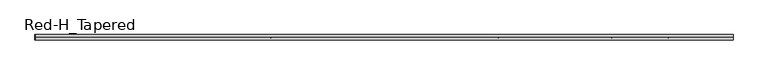
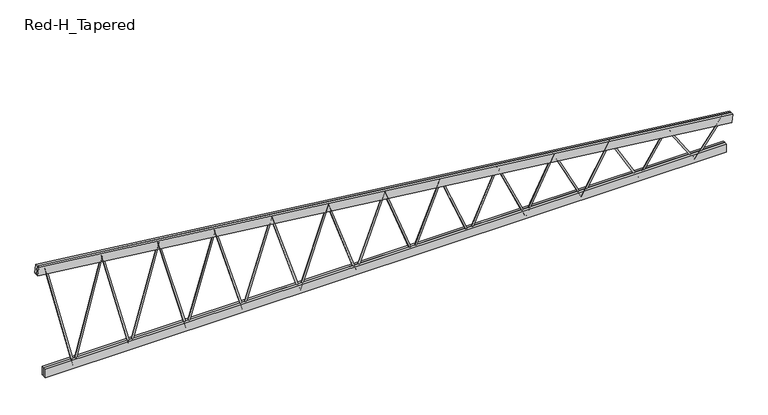
"""IFC4 building model written with IfcOpenShell, lengths in millimetres: beam geometry, Construction_Frames_RedBuilt_Openweb_Red-H_Tapered : Red-H_Tapered."""

from ifc_helpers import new_model, si_unit, point, frame, origin, origin_2d, place, context, project, spatial, polyline, circle_curve, trimmed, segment, composite_curve, outline, extrude, source, transform, mapped, element, save


def red_h_tapered_f2622887(model_context):
    return source(origin(), model_context, "Body", "SweptSolid", [
        extrude(outline(composite_curve([segment(trimmed(circle_curve(origin_2d(), 12.7), [point((0.0, -12.7000001))], [point((0.0, 12.6999999))], False, "CARTESIAN"), True, "CONTINUOUS"), segment(trimmed(circle_curve(origin_2d(), 12.7), [point((0.0, 12.6999999))], [point((0.0, -12.7000001))], False, "CARTESIAN"), True, "CONTINUOUS")], self_intersect=False)), frame((-450.1223958, 0.0, -367.0101562), z_axis=(-0.32912844274512754, 0.0, 0.9442851625309843), x_axis=(0.0, -1.0, 0.0)), (0.0, 0.0, 1.0), 1367.6192555),
        extrude(outline(composite_curve([segment(trimmed(circle_curve(origin_2d(), 12.7), [point((0.0, 12.7000001))], [point((0.0, -12.7))], False, "CARTESIAN"), True, "CONTINUOUS"), segment(trimmed(circle_curve(origin_2d(), 12.7), [point((0.0, -12.7))], [point((0.0, 12.7000001))], False, "CARTESIAN"), True, "CONTINUOUS")], self_intersect=False)), frame((-1350.3671875, 0.0, -367.0101562), z_axis=(0.3291284427451277, 0.0, 0.9442851625309842), x_axis=(0.0, -1.0, 0.0)), (0.0, 0.0, 1.0), 1367.6192555),
        extrude(outline(composite_curve([segment(trimmed(circle_curve(origin_2d(), 12.7), [point((0.0, -12.7))], [point((0.0, 12.7))], False, "CARTESIAN"), True, "CONTINUOUS"), segment(trimmed(circle_curve(origin_2d(), 12.7), [point((0.0, 12.7))], [point((0.0, -12.7))], False, "CARTESIAN"), True, "CONTINUOUS")], self_intersect=False)), frame((-1350.3671875, 0.0, -367.0101562), z_axis=(-0.3075867291849269, 0.0, 0.9515200491998677), x_axis=(0.0, -1.0, 0.0)), (0.0, 0.0, 1.0), 1463.3999231),
        extrude(outline(composite_curve([segment(trimmed(circle_curve(origin_2d(), 12.7), [point((0.0, -12.7))], [point((0.0, 12.7000001))], False, "CARTESIAN"), True, "CONTINUOUS"), segment(trimmed(circle_curve(origin_2d(), 12.7), [point((0.0, 12.7000001))], [point((0.0, -12.7))], False, "CARTESIAN"), True, "CONTINUOUS")], self_intersect=False)), frame((-2250.6119792, 0.0, -367.0101562), z_axis=(0.3075867291849308, 0.0, 0.9515200491998664), x_axis=(0.0, -1.0, 0.0)), (0.0, 0.0, 1.0), 1463.3999231),
        extrude(outline(composite_curve([segment(trimmed(circle_curve(origin_2d(), 12.7), [point((0.0, 12.7))], [point((0.0, -12.7))], False, "CARTESIAN"), True, "CONTINUOUS"), segment(trimmed(circle_curve(origin_2d(), 12.7), [point((0.0, -12.7))], [point((0.0, 12.7))], False, "CARTESIAN"), True, "CONTINUOUS")], self_intersect=False)), frame((-2250.6119792, 0.0, -367.0101562), z_axis=(-0.28856898556555155, 0.0, 0.9574591064738318), x_axis=(0.0, -1.0, 0.0)), (0.0, 0.0, 1.0), 1559.84329),
        extrude(outline(composite_curve([segment(trimmed(circle_curve(origin_2d(), 12.7), [point((0.0, -12.7))], [point((0.0, 12.7))], False, "CARTESIAN"), True, "CONTINUOUS"), segment(trimmed(circle_curve(origin_2d(), 12.7), [point((0.0, 12.7))], [point((0.0, -12.7))], False, "CARTESIAN"), True, "CONTINUOUS")], self_intersect=False)), frame((-3150.8567708, 0.0, -367.0101562), z_axis=(0.28856898556555044, 0.0, 0.9574591064738323), x_axis=(0.0, -1.0, 0.0)), (0.0, 0.0, 1.0), 1559.84329),
        extrude(outline(composite_curve([segment(trimmed(circle_curve(origin_2d(), 12.7), [point((0.0, 12.7))], [point((0.0, -12.7000001))], False, "CARTESIAN"), True, "CONTINUOUS"), segment(trimmed(circle_curve(origin_2d(), 12.7), [point((0.0, -12.7000001))], [point((0.0, 12.7))], False, "CARTESIAN"), True, "CONTINUOUS")], self_intersect=False)), frame((-3150.8567708, 0.0, -367.0101562), z_axis=(-0.2716762785065164, 0.0, 0.9623886947054447), x_axis=(0.0, -1.0, 0.0)), (0.0, 0.0, 1.0), 1656.8336342),
        extrude(outline(composite_curve([segment(trimmed(circle_curve(origin_2d(), 12.7), [point((0.0, -12.7))], [point((0.0, 12.7))], False, "CARTESIAN"), True, "CONTINUOUS"), segment(trimmed(circle_curve(origin_2d(), 12.7), [point((0.0, 12.7))], [point((0.0, -12.7))], False, "CARTESIAN"), True, "CONTINUOUS")], self_intersect=False)), frame((-4051.1015625, 0.0, -367.0101562), z_axis=(0.27167627850652204, 0.0, 0.9623886947054432), x_axis=(0.0, -1.0, 0.0)), (0.0, 0.0, 1.0), 1656.8336342),
        extrude(outline(composite_curve([segment(trimmed(circle_curve(origin_2d(), 12.7), [point((0.0, 12.7))], [point((0.0, -12.7))], False, "CARTESIAN"), True, "CONTINUOUS"), segment(trimmed(circle_curve(origin_2d(), 12.7), [point((0.0, -12.7))], [point((0.0, 12.7))], False, "CARTESIAN"), True, "CONTINUOUS")], self_intersect=False)), frame((-4051.1015625, 0.0, -367.0101562), z_axis=(-0.25658522909134096, 0.0, 0.9665216087662728), x_axis=(0.0, -1.0, 0.0)), (0.0, 0.0, 1.0), 1754.2802344),
        extrude(outline(composite_curve([segment(trimmed(circle_curve(origin_2d(), 12.7), [point((0.0, -12.7))], [point((0.0, 12.7000001))], False, "CARTESIAN"), True, "CONTINUOUS"), segment(trimmed(circle_curve(origin_2d(), 12.7), [point((0.0, 12.7000001))], [point((0.0, -12.7))], False, "CARTESIAN"), True, "CONTINUOUS")], self_intersect=False)), frame((-4951.3463542, 0.0, -367.0101562), z_axis=(0.2565852290913401, 0.0, 0.966521608766273), x_axis=(0.0, -1.0, 0.0)), (0.0, 0.0, 1.0), 1754.2802344),
        extrude(outline(composite_curve([segment(trimmed(circle_curve(origin_2d(), 12.7), [point((0.0, 12.7))], [point((0.0, -12.7))], False, "CARTESIAN"), True, "CONTINUOUS"), segment(trimmed(circle_curve(origin_2d(), 12.7), [point((0.0, -12.7))], [point((0.0, 12.7))], False, "CARTESIAN"), True, "CONTINUOUS")], self_intersect=False)), frame((-4951.3463542, 0.0, -367.0101562), z_axis=(-0.24303207386708506, 0.0, 0.9700182529580893), x_axis=(0.0, -1.0, 0.0)), (0.0, 0.0, 1.0), 1852.111076),
        extrude(outline(composite_curve([segment(trimmed(circle_curve(origin_2d(), 12.7), [point((0.0, 12.7))], [point((0.0, -12.7))], False, "CARTESIAN"), True, "CONTINUOUS"), segment(trimmed(circle_curve(origin_2d(), 12.7), [point((0.0, -12.7))], [point((0.0, 12.7))], False, "CARTESIAN"), True, "CONTINUOUS")], self_intersect=False)), frame((4951.3463542, 0.0, -367.0101562), z_axis=(0.6103390645889434, 0.0, 0.7921402819177256), x_axis=(0.0, -1.0, 0.0)), (0.0, 0.0, 1.0), 737.4956347),
        extrude(outline(composite_curve([segment(trimmed(circle_curve(origin_2d(), 12.7), [point((0.0, -12.7000001))], [point((0.0, 12.7))], False, "CARTESIAN"), True, "CONTINUOUS"), segment(trimmed(circle_curve(origin_2d(), 12.7), [point((0.0, 12.7))], [point((0.0, -12.7000001))], False, "CARTESIAN"), True, "CONTINUOUS")], self_intersect=False)), frame((4951.3463542, 0.0, -367.0101562), z_axis=(-0.5490306886626473, 0.0, 0.8358021912549759), x_axis=(0.0, -1.0, 0.0)), (0.0, 0.0, 1.0), 819.8492455),
        extrude(outline(composite_curve([segment(trimmed(circle_curve(origin_2d(), 12.7), [point((0.0, 12.7))], [point((0.0, -12.7))], False, "CARTESIAN"), True, "CONTINUOUS"), segment(trimmed(circle_curve(origin_2d(), 12.7), [point((0.0, -12.7))], [point((0.0, 12.7))], False, "CARTESIAN"), True, "CONTINUOUS")], self_intersect=False)), frame((4051.1015625, 0.0, -367.0101562), z_axis=(0.5490306886626476, 0.0, 0.8358021912549758), x_axis=(0.0, -1.0, 0.0)), (0.0, 0.0, 1.0), 819.8492455),
        extrude(outline(composite_curve([segment(trimmed(circle_curve(origin_2d(), 12.7), [point((0.0, -12.7))], [point((0.0, 12.7))], False, "CARTESIAN"), True, "CONTINUOUS"), segment(trimmed(circle_curve(origin_2d(), 12.7), [point((0.0, 12.7))], [point((0.0, -12.7))], False, "CARTESIAN"), True, "CONTINUOUS")], self_intersect=False)), frame((4051.1015625, 0.0, -367.0101562), z_axis=(-0.4968284949921359, 0.0, 0.8678487463630107), x_axis=(0.0, -1.0, 0.0)), (0.0, 0.0, 1.0), 905.9915049),
        extrude(outline(composite_curve([segment(trimmed(circle_curve(origin_2d(), 12.7), [point((0.0, 12.7))], [point((0.0, -12.6999999))], False, "CARTESIAN"), True, "CONTINUOUS"), segment(trimmed(circle_curve(origin_2d(), 12.7), [point((0.0, -12.6999999))], [point((0.0, 12.7))], False, "CARTESIAN"), True, "CONTINUOUS")], self_intersect=False)), frame((3150.8567708, 0.0, -367.0101562), z_axis=(0.4968284949921344, 0.0, 0.8678487463630115), x_axis=(0.0, -1.0, 0.0)), (0.0, 0.0, 1.0), 905.9915049),
        extrude(outline(composite_curve([segment(trimmed(circle_curve(origin_2d(), 12.7), [point((0.0, -12.7))], [point((0.0, 12.7))], False, "CARTESIAN"), True, "CONTINUOUS"), segment(trimmed(circle_curve(origin_2d(), 12.7), [point((0.0, 12.7))], [point((0.0, -12.7))], False, "CARTESIAN"), True, "CONTINUOUS")], self_intersect=False)), frame((3150.8567708, 0.0, -367.0101562), z_axis=(-0.4524121304058867, 0.0, 0.8918089841785667), x_axis=(0.0, -1.0, 0.0)), (0.0, 0.0, 1.0), 994.9388303),
        extrude(outline(composite_curve([segment(trimmed(circle_curve(origin_2d(), 12.7), [point((0.0, 12.7))], [point((0.0, -12.7))], False, "CARTESIAN"), True, "CONTINUOUS"), segment(trimmed(circle_curve(origin_2d(), 12.7), [point((0.0, -12.7))], [point((0.0, 12.7))], False, "CARTESIAN"), True, "CONTINUOUS")], self_intersect=False)), frame((2250.6119792, 0.0, -367.0101562), z_axis=(0.4524121304058875, 0.0, 0.8918089841785662), x_axis=(0.0, -1.0, 0.0)), (0.0, 0.0, 1.0), 994.9388303),
        extrude(outline(composite_curve([segment(trimmed(circle_curve(origin_2d(), 12.7), [point((0.0, -12.7))], [point((0.0, 12.6999999))], False, "CARTESIAN"), True, "CONTINUOUS"), segment(trimmed(circle_curve(origin_2d(), 12.7), [point((0.0, 12.6999999))], [point((0.0, -12.7))], False, "CARTESIAN"), True, "CONTINUOUS")], self_intersect=False)), frame((2250.6119792, 0.0, -367.0101562), z_axis=(-0.414476502078826, 0.0, 0.9100600140784678), x_axis=(0.0, -1.0, 0.0)), (0.0, 0.0, 1.0), 1086.0022066),
        extrude(outline(composite_curve([segment(trimmed(circle_curve(origin_2d(), 12.7), [point((0.0, 12.7))], [point((0.0, -12.7))], False, "CARTESIAN"), True, "CONTINUOUS"), segment(trimmed(circle_curve(origin_2d(), 12.7), [point((0.0, -12.7))], [point((0.0, 12.7))], False, "CARTESIAN"), True, "CONTINUOUS")], self_intersect=False)), frame((1350.3671875, 0.0, -367.0101562), z_axis=(0.4144765020788303, 0.0, 0.9100600140784658), x_axis=(0.0, -1.0, 0.0)), (0.0, 0.0, 1.0), 1086.0022066),
        extrude(outline(composite_curve([segment(trimmed(circle_curve(origin_2d(), 12.7), [point((0.0, -12.7))], [point((0.0, 12.7))], False, "CARTESIAN"), True, "CONTINUOUS"), segment(trimmed(circle_curve(origin_2d(), 12.7), [point((0.0, 12.7))], [point((0.0, -12.7))], False, "CARTESIAN"), True, "CONTINUOUS")], self_intersect=False)), frame((1350.3671875, 0.0, -367.0101562), z_axis=(-0.3818831951022662, 0.0, 0.9242105957510358), x_axis=(0.0, -1.0, 0.0)), (0.0, 0.0, 1.0), 1178.6912899),
        extrude(outline(composite_curve([segment(trimmed(circle_curve(origin_2d(), 12.7), [point((0.0, 12.7))], [point((0.0, -12.6999999))], False, "CARTESIAN"), True, "CONTINUOUS"), segment(trimmed(circle_curve(origin_2d(), 12.7), [point((0.0, -12.6999999))], [point((0.0, 12.7))], False, "CARTESIAN"), True, "CONTINUOUS")], self_intersect=False)), frame((450.1223958, 0.0, -367.0101562), z_axis=(0.3818831951022686, 0.0, 0.9242105957510348), x_axis=(0.0, -1.0, 0.0)), (0.0, 0.0, 1.0), 1178.6912899),
        extrude(outline(composite_curve([segment(trimmed(circle_curve(origin_2d(), 12.7), [point((0.0, -12.7))], [point((0.0, 12.7))], False, "CARTESIAN"), True, "CONTINUOUS"), segment(trimmed(circle_curve(origin_2d(), 12.7), [point((0.0, 12.7))], [point((0.0, -12.7))], False, "CARTESIAN"), True, "CONTINUOUS")], self_intersect=False)), frame((450.1223958, 0.0, -367.0101562), z_axis=(-0.35368881452865064, 0.0, 0.935363150053132), x_axis=(0.0, -1.0, 0.0)), (0.0, 0.0, 1.0), 1272.6509218),
        extrude(outline(composite_curve([segment(trimmed(circle_curve(origin_2d(), 12.7), [point((0.0, 12.7))], [point((0.0, -12.7))], False, "CARTESIAN"), True, "CONTINUOUS"), segment(trimmed(circle_curve(origin_2d(), 12.7), [point((0.0, -12.7))], [point((0.0, 12.7))], False, "CARTESIAN"), True, "CONTINUOUS")], self_intersect=False)), frame((-450.1223958, 0.0, -367.0101562), z_axis=(0.3536888145286179, 0.0, 0.9353631500531443), x_axis=(0.0, -1.0, 0.0)), (0.0, 0.0, 1.0), 1272.6509218),
        extrude(outline(polyline([(-5426.86875, -41.275), (-5426.86875, -3.175), (5426.86875, -3.175), (5426.86875, -41.275), (-5426.86875, -41.275)])), frame((0.0, 0.0, -386.0601562), z_axis=(0.0, 0.0, 1.0), x_axis=(1.0, 0.0, 0.0)), (0.0, 0.0, 1.0), 139.7),
        extrude(outline(polyline([(-5426.86875, 3.175), (-5426.86875, 41.275), (5426.86875, 41.275), (5426.86875, 3.175), (-5426.86875, 3.175)])), frame((0.0, 0.0, -386.0601562), z_axis=(0.0, 0.0, 1.0), x_axis=(1.0, 0.0, 0.0)), (0.0, 0.0, 1.0), 139.7),
        extrude(outline(polyline([(0.0, -38.1), (0.0, 0.0), (11131.0909694, 0.0), (11131.0909694, -38.1), (0.0, -38.1)])), frame((-5544.5671891, -3.175, 1367.4705018), z_axis=(0.11523578448213238, 0.0, 0.9933381669777859), x_axis=(0.9933381669777859, 0.0, -0.11523578448213238)), (0.0, 0.0, 1.0), 139.7),
        extrude(outline(polyline([(0.0, -38.1), (0.0, 0.0), (11131.0909694, 0.0), (11131.0909694, -38.1), (0.0, -38.1)])), frame((-5544.5671891, 41.275, 1367.4705018), z_axis=(0.11523578448213238, 0.0, 0.9933381669777859), x_axis=(0.9933381669777859, 0.0, -0.11523578448213238)), (0.0, 0.0, 1.0), 139.7),
    ])


if __name__ == "__main__":
    model = new_model("IFC4")
    model_context = context("Model", 3, world=origin())
    ifc_project = project(units=[si_unit("LENGTHUNIT", "METRE", prefix="MILLI")], contexts=[model_context])
    site = spatial("IfcSite", under=ifc_project)
    building = spatial("IfcBuilding", under=site)
    placement = place(None, origin())
    red_h_tapered_shape = red_h_tapered_f2622887(model_context)
    element("IfcBeam", 1, ObjectType="Construction_Frames_RedBuilt_Openweb_Red-H_Tapered : Red-H_Tapered", at=placement, inside=building, context=model_context, shape_type="MappedRepresentation", body=[
        mapped(red_h_tapered_shape, transform((0.0, 0.0, 0.0), x_axis=(1.0, 0.0, 0.0), y_axis=(0.0, 1.0, 0.0), z_axis=(0.0, 0.0, 1.0))),
    ])
    save(model, "model.ifc")

# Revit data of these elements
# Type "Construction_Frames_RedBuilt_Openweb_Red-H_Tapered : Red-H_Tapered"
#   Youtube clip = ""
#   Weight Net (Kg) = "0"
#   Webs = "Up to 2\" diameter tubular steel"
#   Uniformat II Description = ""
#   Uniformat II Code = ""
#   Uniclass 2015 Name = "Softwood trusses"
#   Uniclass 2015 Code = "Pr_20_85_90_81"
#   Uniclass 2.0 Description = "Structural Framing Systems"
#   Uniclass 2.0 Code = "SS-15-10-75"
#   Uniclass 1.4 Description = "Trusses"
#   Uniclass 1.4 Code = "L3523"
#   UNSPSC Code = "30103606"
#   Technical description = "http://www.redbuilt.com/reference/literature-and-other-resources"
#   Region South America = "None"
#   Region Oceania = "None"
#   Region North America = "US"
#   Region Middle East = "None"
#   Region Europe = "None"
#   Region Asia = "None"
#   Region Antarctica = "None"
#   Region Africa = "None"
#   QR code = "http://bimobject.com/redbuilt/product/redbuilt-0003"
#   Product url = "http://www.redbuilt.com/products/default.aspx?id=2"
#   Product group = "Wood Trusses"
#   Product family = "Construction"
#   Product data url = "https://bimobject.com/redbuilt/product/redbuilt-0003"
#   Product certification = ""
#   Product SKU = "redbuilt-0003"
#   Product Page URL = "http://www.redbuilt.com/commercial-systems/red-m-red-h-open-web-trusses"
#   Product Guid = "2c5793f2-6ffb-4665-b825-cf90c048e711"
#   Product Documentation Link = "http://www.redbuilt.com/documents/OW_Guide_2017_07_LowRes_wLinks.pdf"
#   OmniClass Description = "Wood Trusses"
#   OmniClass Code = "23-13 35 19 13 17"
#   NBS Reference Description = ""
#   NBS Reference Code = ""
#   Material secondary = "Steel"
#   Material main = "Wood"
#   Masterformat 2014 Description = "Metal-Web Wood Joists"
#   Masterformat 2014 Code = "06 17 36"
#   Manufacturer name = "RedBuilt"
#   Manufacturer country = "United States"
#   Installation instructions = "http://www.redbuilt.com/documents/Installation_Sheets_Open-Web.pdf"
#   IFC Classification = ""
#   EAN code = ""
#   Design country = "United States"
#   Product Information = "http://redbuilt.com/products/default.aspx?id=2"
#   Model = "Red-H-Tapered"
#   Manufacturer URL = "http://redbuilt.com/"
#   Manufacturer = "RedBuilt™"
#   Description = "Open Web Truss"
#   Date of publishing = "8/17/2010"
#   Contact us = "http://redbuilt.com/contact/"
#   Chords = "Double 1½\" x 5½\" MSR lumber"
#   COBIe Type Category = ""
#   Brand url = "http://www.redbuilt.com"
#   BIMobject main category code = "construction"
#   BIMobject main category = "Construction"
#   BIMobject category code = "construction-frames-trusses"
#   BIMobject category = "Frames & Trusses"
#   Web Radius = 0' - 0 1/2"
#   Web Layout Offset Start [instance default] = 0' - 5"
#   Web Layout Offset End [instance default] = 0' - 5"
#   Web Diameter = 0' - 1"
#   TotalLength [instance default] = 20' - 0"
#   Span Minimum = 4' - 0"
#   Span Maximum = 70' - 0"
#   Span Limit [instance default] = 20' - 0"
#   Nominal width = 0' - 0"
#   Nominal height = 0' - 0"
#   Inner Depth Top [instance default] = 0' - 2.76372"
#   Depth Start [instance default] = 6' - 0"
#   Top Chord Length [instance default] = 20' - 1.19701"
#   TC Extension Start Aux [instance default] = 0' - 0"
#   TC Extension End Aux [instance default] = 0' - 0"
#   T-B Chord Length Difference L [instance default] = 0' - 4"
#   T-B Chord Length Difference [instance default] = 0' - 4"
#   Height 2 [instance default] = 6' - 0"
#   Depth Minimum at Wall = 2' - 0"
#   Depth Maximum at Wall = 6' - 0"
#   Depth Lower End [instance default] = 2' - 0"
#   Depth Higher End [instance default] = 6' - 0"
#   Depth End [instance default] = 2' - 0"
#   Depth 2 [instance default] = 2' - 0"
#   Chord Width = 0' - 3 1/4"
#   Chord Thickness = 0' - 1 1/2"
#   Chord Depth = 0' - 5 1/2"
#   Offset Start [instance default] = 0' - 0"
#   TC Extension Start [instance default] = 0' - 0"
#   End Panel = 0' - 5"
#   Offset End [instance default] = 0' - 0"
#   TC Extension End [instance default] = 0' - 0"
#   Length [instance default] = 20' - 0"
#   Angle [instance default] = 5.71059°
#   Span Limit Warning [instance default] = no
#   Edition number = 1
#   Top Bearing Start [instance default] = yes
#   Top Bearing End [instance default] = yes
#   Bottom Bearing Start [instance default] = no
#   Bottom Bearing End [instance default] = no
#   8 Panels [instance default] = yes
#   16 Panels [instance default] = no
#   12 Panels [instance default] = no
#   Web Material = RedBuilt-Steel, Galvanized
#   Clip Material = RedBuilt-Steel, Galvanized
#   Chords Material = RedBuilt-MSR
#   URL = ""
#   Assembly Code = ""
# Element 1 (IfcBeam, "Construction_Frames_RedBuilt_Openweb_Red-H_Tapered : Red-H_Tapered")
#   TotalLength = 36' - 3 5/16"
#   Span Limit = 36' - 3 5/16"
#   Inner Depth Top = 0' - 2.76844"
#   Top Chord Length = 36' - 6.23193"
#   Depth 2 = 4' - 2 1/2"
#   Angle = 6.61722°
#   8 Panels = no
#   12 Panels = yes
#   Materials on its faces: "RedBuilt-Steel, Galvanized", "RedBuilt-MSR"
# Materials
#   "RedBuilt-Steel, Galvanized": class "Metal", colour RGB 164 172 176, transparency 0, Manufacturer = "RedBuilt. LLC", Comments = "Openweb Metal Web", URL = "http://www.redbuilt.com/", Description = "Galvanized steel", Cost = 0
#   "RedBuilt-MSR": class "Wood", colour RGB 213 182 136, transparency 0, Manufacturer = "RedBuilt, LLC", URL = "http://www.redbuilt.com/", Cost = 0
